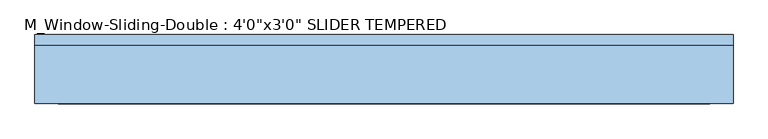
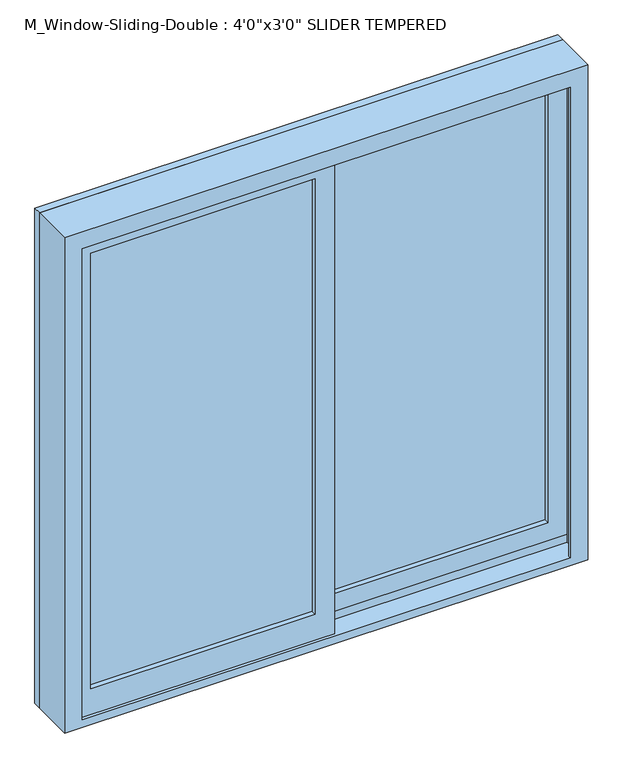
"""IFC4 building model written with IfcOpenShell, lengths in millimetres: window geometry."""

from ifc_helpers import new_model, si_unit, frame, origin, place, context, project, spatial, polyline, outline, extrude, faceted_brep, source, transform, mapped, element, save


def window_ab087c2d(model_context):
    return source(origin(), model_context, "Body", "SolidModel", [
        faceted_brep([(-609.6, 35.56, 900.0), (609.6, 35.56, 900.0), (609.6, -66.04, 900.0), (-609.6, -66.04, 900.0), (-568.6778905, -66.04, 2078.2778905), (-568.6778905, -66.04, 919.05), (-568.6778905, -59.69, 919.05), (-568.6778905, -59.69, 2078.2778905), (-590.55, -59.69, 919.05), (-590.55, -59.69, 2100.15), (590.55, -59.69, 2100.15), (590.55, -59.69, 919.05), (568.6778905, -59.69, 919.05), (568.6778905, -59.69, 2078.2778905), (-590.55, -15.24, 919.05), (-590.55, -15.24, 938.1), (-590.55, 29.21, 938.1), (-590.55, 29.21, 919.05), (-590.55, 35.56, 919.05), (-590.55, 35.56, 2100.15), (-609.6, 35.56, 2119.2), (609.6, 35.56, 2119.2), (590.55, 35.56, 2100.15), (590.55, 35.56, 919.05), (-609.6, -66.04, 2119.2), (609.6, -66.04, 2119.2), (568.6778905, -66.04, 2078.2778905), (568.6778905, -66.04, 919.05), (590.55, 29.21, 919.05), (590.55, 29.21, 938.1), (590.55, -15.24, 938.1), (590.55, -15.24, 919.05)], [[[0, 1, 2, 3]], [[4, 5, 6, 7]], [[7, 6, 8, 9, 10, 11, 12, 13]], [[9, 8, 14, 15, 16, 17, 18, 19]], [[0, 20, 21, 1], [22, 19, 18, 23]], [[24, 20, 0, 3]], [[2, 25, 24, 3], [4, 26, 27, 5]], [[7, 13, 26, 4]], [[9, 19, 22, 10]], [[20, 24, 25, 21]], [[13, 12, 27, 26]], [[22, 23, 28, 29, 30, 31, 11, 10]], [[21, 25, 2, 1]], [[27, 12, 11, 31, 14, 8, 6, 5]], [[31, 30, 15, 14]], [[30, 29, 16, 15]], [[29, 28, 17, 16]], [[18, 17, 28, 23]]]),
        extrude(outline(polyline([(2119.2, 609.6), (2119.2, -609.6), (900.0, -609.6), (900.0, 609.6), (2119.2, 609.6)]), holes=[polyline([(2100.15, -590.55), (2100.15, 590.55), (919.05, 590.55), (919.05, -590.55), (2100.15, -590.55)])]), frame((0.0, 35.56, 0.0), z_axis=(0.0, 1.0, 0.0), x_axis=(0.0, 0.0, 1.0)), (0.0, 0.0, 1.0), 19.05),
        extrude(outline(polyline([(546.1, -2.54), (22.225, -2.54), (22.225, 3.81), (546.1, 3.81), (546.1, -2.54)])), frame((0.0, 0.0, 982.55), z_axis=(0.0, 0.0, 1.0), x_axis=(1.0, 0.0, 0.0)), (0.0, 0.0, 1.0), 1073.15),
        extrude(outline(polyline([(546.1, 10.16), (22.225, 10.16), (22.225, 16.51), (546.1, 16.51), (546.1, 10.16)])), frame((0.0, 0.0, 982.55), z_axis=(0.0, 0.0, 1.0), x_axis=(1.0, 0.0, 0.0)), (0.0, 0.0, 1.0), 1073.15),
        extrude(outline(polyline([(-22.225, -46.99), (-546.1, -46.99), (-546.1, -40.64), (-22.225, -40.64), (-22.225, -46.99)])), frame((0.0, 0.0, 982.55), z_axis=(0.0, 0.0, 1.0), x_axis=(1.0, 0.0, 0.0)), (0.0, 0.0, 1.0), 1073.15),
        extrude(outline(polyline([(-22.225, -34.29), (-546.1, -34.29), (-546.1, -27.94), (-22.225, -27.94), (-22.225, -34.29)])), frame((0.0, 0.0, 982.55), z_axis=(0.0, 0.0, 1.0), x_axis=(1.0, 0.0, 0.0)), (0.0, 0.0, 1.0), 1073.15),
        extrude(outline(polyline([(919.05, 22.225), (2100.15, 22.225), (2100.15, -590.55), (919.05, -590.55), (919.05, 22.225)]), holes=[polyline([(2055.7, -546.1), (2055.7, -22.225), (982.55, -22.225), (982.55, -546.1), (2055.7, -546.1)])]), frame((0.0, -59.69, 0.0), z_axis=(0.0, 1.0, 0.0), x_axis=(0.0, 0.0, 1.0)), (0.0, 0.0, 1.0), 44.45),
        extrude(outline(polyline([(938.1, -22.225), (938.1, 590.55), (2100.15, 590.55), (2100.15, -22.225), (938.1, -22.225)]), holes=[polyline([(982.55, 546.1), (982.55, 22.225), (2055.7, 22.225), (2055.7, 546.1), (982.55, 546.1)])]), frame((0.0, -15.24, 0.0), z_axis=(0.0, 1.0, 0.0), x_axis=(0.0, 0.0, 1.0)), (0.0, 0.0, 1.0), 44.45),
    ])


if __name__ == "__main__":
    model = new_model("IFC4")
    model_context = context("Model", 3, world=origin())
    ifc_project = project(units=[si_unit("LENGTHUNIT", "METRE", prefix="MILLI")], contexts=[model_context])
    site = spatial("IfcSite", under=ifc_project)
    building = spatial("IfcBuilding", under=site)
    placement = place(None, origin())
    window_shape = window_ab087c2d(model_context)
    element("IfcWindow", 1, ObjectType="M_Window-Sliding-Double : 4'0\"x3'0\" SLIDER TEMPERED", at=placement, inside=building, context=model_context, shape_type="MappedRepresentation", body=[
        mapped(window_shape, transform((0.0, 0.0, 0.0), x_axis=(1.0, 0.0, 0.0), y_axis=(0.0, 1.0, 0.0), z_axis=(0.0, 0.0, 1.0))),
    ])
    save(model, "model.ifc")

# Revit data of these elements
# Type "M_Window-Sliding-Double : 4'0\"x3'0\" SLIDER TEMPERED"
#   Type Mark = "5"
#   Fire Rating = "0.5h"
#   Assembly Code = "B2020100"
#   Analytic Construction = "Double glazing - domestic"
#   Window Inset [instance default] = 0' - 0"
#   Wall Thickness [instance default] = 0' - 5.90551"
#   Visual Light Transmittance = 0.81
#   Thermal Resistance (R) = 1.8146 (h·ft²·°F)/BTU
#   Solar Heat Gain Coefficient = 0.76
#   Muntin Width = 1' - 8 5/8"
#   Muntin Height = 3' - 6 1/4"
#   Interior Wall Closure [instance default] = 0' - 2.65551"
#   Heat Transfer Coefficient (U) = 0.5511 BTU/(h·ft²·°F)
#   Frame Extension [instance default] = 0' - 0 1/4"
#   Exterior Wall Closure [instance default] = 0' - 1 1/4"
#   Rough Width = 4' - 0.59055"
#   Rough Height = 4' - 0.59055"
#   Height = 4' - 0"
#   Extension Jamb [instance default] = 0' - 2.65551"
#   Default Sill Height = 2' - 11.43307"
#   Width = 4' - 0"
#   Interior Trim Visibility [instance default] = yes
#   Indicator Visibility [instance default] = yes
#   Exterior Trim Visibility [instance default] = yes
#   Muntin Visibility = yes
#   Extension Jamb Visibility [instance default] = yes
#   Muntin Pattern = M_Muntin Pattern_2x2 : M_Muntin Pattern_2x2
#   Interior Trim Material = Wood - Stained
#   Interior Trim = M_Trim-Window-Interior-Flat : Picture Frame
#   Interior Frame Material = Wood - Stained
#   Glass Panel Material = Glass
#   Exterior Trim Material = Clad - White
#   Exterior Trim = M_Trim-Window-Exterior-Flat : with Sill
#   Exterior Frame Material = Clad - White
#   Wall Closure = (empty or 0)
# Element 1 (IfcWindow, "M_Window-Sliding-Double : 4'0\"x3'0\" SLIDER TEMPERED")
#   Wall Thickness = 0' - 4"
#   Extension Jamb = 0' - 0 3/4"
#   Materials on its faces: "Wood - Stained", "Glass", "Clad - White"
# Materials
#   "Wood - Stained": class "Wood", colour RGB 224 178 126, transparency 0, Cost = 0
#   "Glass": class "Glass", colour RGB 0 128 192, transparency 0.75, Description = "Soda Lime Glass", Cost = 0
#   "Clad - White": class "Wood", colour RGB 242 242 238, transparency 0, Cost = 0
